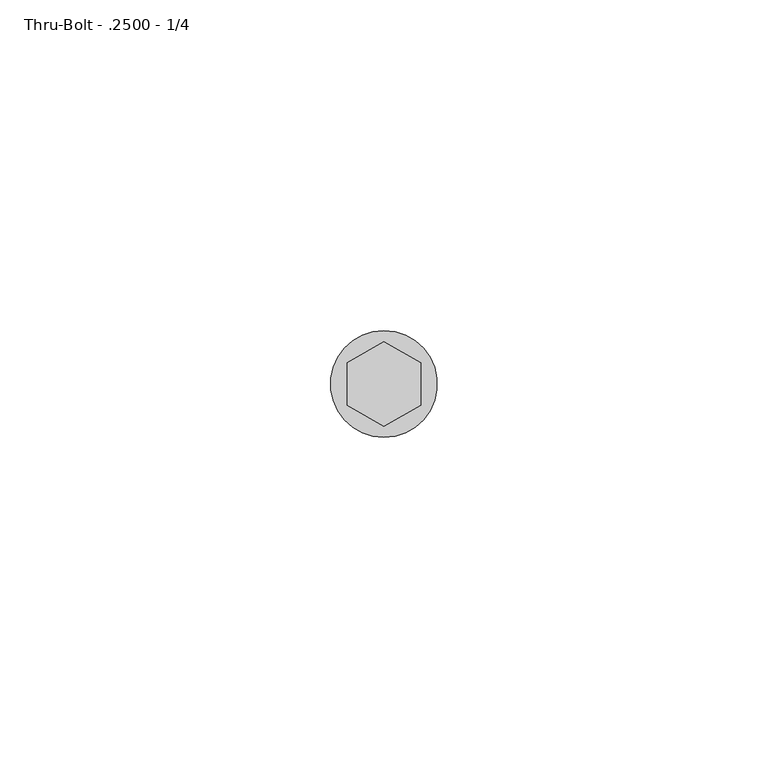
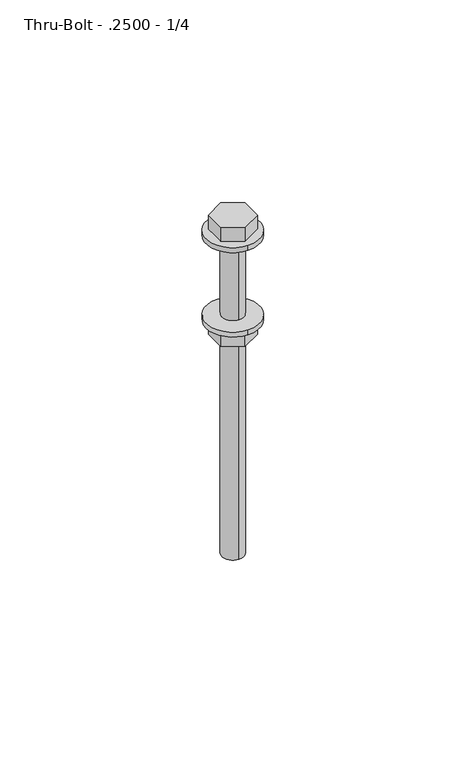
"""IFC4 building model written with IfcOpenShell, lengths in millimetres: fastener geometry, 060523 - W_P_C - Fastenings - Generic : Thru-Bolt - .2500 - 1/4."""

from ifc_helpers import new_model, si_unit, point, frame, origin, origin_with_axes, origin_2d, place, context, project, spatial, polyline, circle_curve, trimmed, segment, composite_curve, outline, extrude, source, transform, mapped, element, save


def thru_bolt_2500_1_4_d93b7c06(model_context):
    return source(origin(), model_context, "Body", "SweptSolid", [
        extrude(outline(composite_curve([segment(trimmed(circle_curve(origin_2d(), 8.0645), [point((0.0, 8.0645))], [point((0.0, -8.0645))], False, "CARTESIAN"), True, "CONTINUOUS"), segment(trimmed(circle_curve(origin_2d(), 8.0645), [point((0.0, -8.0645))], [point((0.0, 8.0645))], False, "CARTESIAN"), True, "CONTINUOUS")], self_intersect=False)), origin_with_axes(), (0.0, 0.0, 1.0), 1.5875),
        extrude(outline(composite_curve([segment(trimmed(circle_curve(origin_2d(), 8.0645), [point((0.0, 8.0645))], [point((0.0, -8.0645))], False, "CARTESIAN"), True, "CONTINUOUS"), segment(trimmed(circle_curve(origin_2d(), 8.0645), [point((0.0, -8.0645))], [point((0.0, 8.0645))], False, "CARTESIAN"), True, "CONTINUOUS")], self_intersect=False)), frame((0.0, 0.0, -26.9875), z_axis=(0.0, 0.0, 1.0), x_axis=(1.0, 0.0, 0.0)), (0.0, 0.0, 1.0), 1.5875),
        extrude(outline(polyline([(-5.55625, -3.2079024), (-5.55625, 3.2079024), (0.0, 6.4158049), (5.55625, 3.2079024), (5.55625, -3.2079024), (0.0, -6.4158049), (-5.55625, -3.2079024)])), frame((0.0, 0.0, -31.75), z_axis=(0.0, 0.0, 1.0), x_axis=(1.0, 0.0, 0.0)), (0.0, 0.0, 1.0), 4.7625),
        extrude(outline(polyline([(-5.55625, 3.2079024), (0.0, 6.4158049), (5.55625, 3.2079024), (5.55625, -3.2079024), (0.0, -6.4158049), (-5.55625, -3.2079024), (-5.55625, 3.2079024)])), frame((0.0, 0.0, 1.5875), z_axis=(0.0, 0.0, 1.0), x_axis=(1.0, 0.0, 0.0)), (0.0, 0.0, 1.0), 4.7625),
        extrude(outline(composite_curve([segment(trimmed(circle_curve(origin_2d(), 3.302), [point((0.0, -3.302))], [point((0.0, 3.302))], False, "CARTESIAN"), True, "CONTINUOUS"), segment(trimmed(circle_curve(origin_2d(), 3.302), [point((0.0, 3.302))], [point((0.0, -3.302))], False, "CARTESIAN"), True, "CONTINUOUS")], self_intersect=False)), frame((0.0, 0.0, -101.6), z_axis=(0.0, 0.0, 1.0), x_axis=(1.0, 0.0, 0.0)), (0.0, 0.0, 1.0), 103.1875),
    ])


if __name__ == "__main__":
    model = new_model("IFC4")
    model_context = context("Model", 3, world=origin())
    ifc_project = project(units=[si_unit("LENGTHUNIT", "METRE", prefix="MILLI")], contexts=[model_context])
    site = spatial("IfcSite", under=ifc_project)
    building = spatial("IfcBuilding", under=site)
    placement = place(None, origin())
    thru_bolt_2500_1_4_shape = thru_bolt_2500_1_4_d93b7c06(model_context)
    element("IfcFastener", 1, ObjectType="060523 - W_P_C - Fastenings - Generic : Thru-Bolt - .2500 - 1/4", at=placement, inside=building, context=model_context, shape_type="MappedRepresentation", body=[
        mapped(thru_bolt_2500_1_4_shape, transform((0.0, 0.0, 0.0), x_axis=(1.0, 0.0, 0.0), y_axis=(0.0, 1.0, 0.0), z_axis=(0.0, 0.0, 1.0))),
    ])
    save(model, "model.ifc")

# Revit data of these elements
# Type "060523 - W_P_C - Fastenings - Generic : Thru-Bolt - .2500 - 1/4"
#   Washer_Thickness = 0' - 0 1/16"
#   Washer Radius = 0' - 0.3175"
#   Washer Offset - Head = 0' - 0 1/16"
#   Washer Offset = 0' - 0 1/16"
#   Thickness_of_Substrate [instance default] = 0' - 1"
#   Side = 0' - 0.25293"
#   Radius = 0' - 0.13"
#   Length [instance default] = 0' - 4"
#   Head Size = 0' - 0 7/16"
#   Head Radius = 0' - 0 7/32"
#   Head Height = 0' - 0 3/16"
#   Double Diameter = 0' - 0.52"
#   Diameter = 0' - 0.26"
#   Default Elevation = 4' - 0"
#   Washer_Nut_Visibility = yes
#   Washer_Head_Visibility = yes
#   Round_Head_Visibility = no
#   Point Visibility = no
#   Nut_Visibility = yes
#   Hex_Head_Visiblilty = yes
#   Washer Material = none
#   Bolt Material (Size) = AT SILL - FASTENER AT 24" O.C.
# Element 1 (IfcFastener, "060523 - W_P_C - Fastenings - Generic : Thru-Bolt - .2500 - 1/4")
#   Materials on its faces: "AT SILL - FASTENER AT 24\" O.C."
# Materials
#   "AT SILL - FASTENER AT 24\" O.C.": class "Generic", colour RGB 120 120 120, transparency 0, Cost = 0
